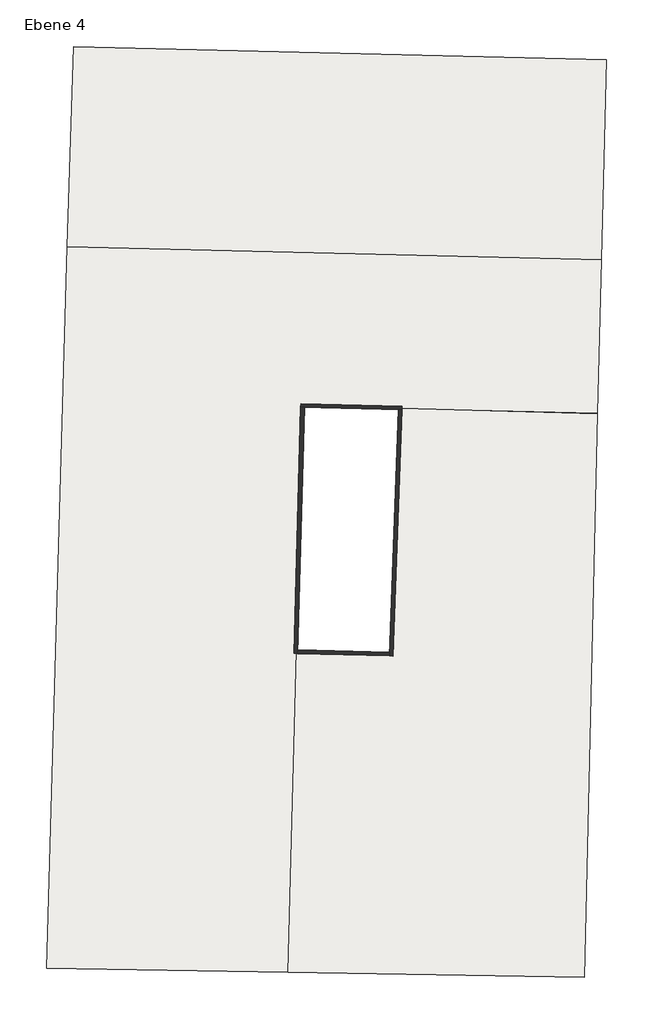
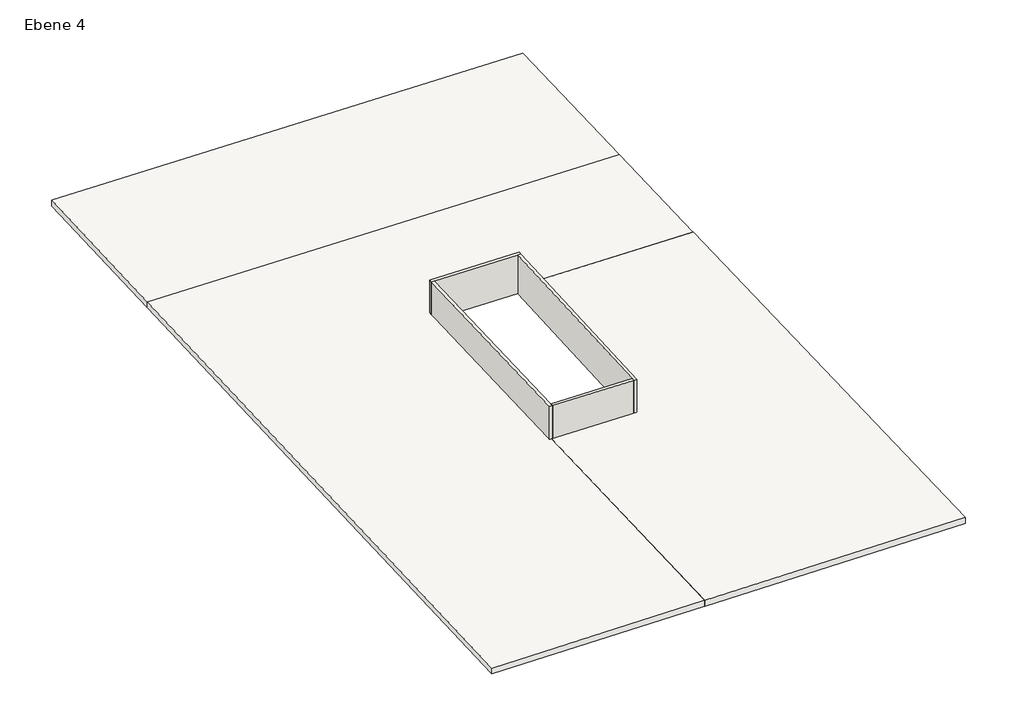
# One storey: 4 walls, 3 slabs.
"""IFC4 building model written with IfcOpenShell, lengths in millimetres."""

from ifc_helpers import new_model, si_unit, frame, origin, place, context, project, spatial, polyline, outline, extrude, faceted_brep, element, save

model = new_model("IFC4")

# Units and contexts
model_context = context("Model", 3, world=origin())
ifc_project = project(units=[si_unit("LENGTHUNIT", "METRE", prefix="MILLI")], contexts=[model_context])

# Site, building, storey
site = spatial("IfcSite", under=ifc_project)
building = spatial("IfcBuilding", under=site)
storey = spatial("IfcBuildingStorey", under=building, Name="Ebene 4", Elevation=3000.0)

# Slabs
placement = place(None, origin())
element("IfcSlab", 1, ObjectType="STB 20.0  FB 10.0 Akustikdecke", at=placement, inside=storey, context=model_context, shape_type="SweptSolid", body=[
    extrude(outline(polyline([(-1151.0631319, -18110.0518993), (-11455.315735, -17930.1905011), (-10568.7895571, 12833.151843), (12212.6461112, 12270.8579117), (12051.1906217, 5729.4608901), (-509.8782218, 6039.4945897), (-1151.0631319, -18110.0518993)])), frame((0.0, 0.0, 3000.0), z_axis=(0.0, 0.0, 1.0), x_axis=(1.0, 0.0, 0.0)), (0.0, 0.0, 1.0), 300.0),
])
element("IfcSlab", 2, ObjectType="STB 20.0  FB 10.0 Akustikdecke", at=placement, inside=storey, context=model_context, shape_type="SweptSolid", body=[
    extrude(outline(polyline([(11494.0304333, -18323.9009543), (-1144.0319966, -18103.302754), (-780.1414101, -4397.7515207), (3237.4967138, -4504.422217), (3618.3842953, 5943.1241384), (12050.8932593, 5719.2359795), (11494.0304333, -18323.9009543)])), frame((0.0, 0.0, 3000.0), z_axis=(0.0, 0.0, 1.0), x_axis=(1.0, 0.0, 0.0)), (0.0, 0.0, 1.0), 300.0),
])
element("IfcSlab", 3, ObjectType="STB 25.0  FB 10.0", at=placement, inside=storey, context=model_context, shape_type="SweptSolid", body=[
    extrude(outline(polyline([(12423.2323245, 20804.9758127), (12212.6461112, 12273.0390386), (-10562.4484458, 12835.1764579), (-10297.2009083, 21365.7640752), (12423.2323245, 20804.9758127)])), frame((0.0, 0.0, 3000.0), z_axis=(0.0, 0.0, 1.0), x_axis=(1.0, 0.0, 0.0)), (0.0, 0.0, 1.0), 300.0),
])

# Walls
element("IfcWall", 4, ObjectType="STB 10.0 + Akustikdecke", at=placement, inside=storey, context=model_context, shape_type="SweptSolid", body=[
    extrude(outline(polyline([(3179.0896913, -4616.4696663), (-735.4392226, -4512.5365812), (-731.4580358, -4362.5894234), (3184.5548982, -4466.5619101), (3179.0896913, -4616.4696663)])), frame((0.0, 0.0, 3000.0), z_axis=(0.0, 0.0, 1.0), x_axis=(1.0, 0.0, 0.0)), (0.0, 0.0, 1.0), 2000.0),
])
element("IfcWall", 5, ObjectType="STB 10.0 + Akustikdecke", at=placement, inside=storey, context=model_context, shape_type="Brep", body=[
    faceted_brep([(3329.0441926, -4620.451048, 3000.0), (3711.7017316, 5875.6443114, 3000.0), (3711.7017316, 5875.6443114, 5000.0), (3329.0441926, -4620.451048, 5000.0), (3179.0896913, -4616.4696663, 3000.0), (3179.0896913, -4616.4696663, 5000.0), (3184.5548982, -4466.5619101, 5000.0), (3561.7472302, 5879.6256932, 5000.0), (3561.7472302, 5879.6256932, 3000.0), (3184.5548982, -4466.5619101, 3000.0)], [[[0, 1, 2, 3]], [[4, 5, 6, 7, 8, 9]], [[0, 3, 5, 4]], [[1, 0, 4, 9, 8]], [[3, 2, 7, 6, 5]], [[2, 1, 8, 7]]]),
])
element("IfcWall", 6, ObjectType="STB 10.0 + Akustikdecke", at=placement, inside=storey, context=model_context, shape_type="Brep", body=[
    faceted_brep([(3717.1669385, 6025.5520677, 3000.0), (-602.6543337, 6140.2459074, 3000.0), (-602.6543337, 6140.2459074, 5000.0), (3717.1669385, 6025.5520677, 5000.0), (3711.7017316, 5875.6443114, 3000.0), (3711.7017316, 5875.6443114, 5000.0), (3561.7472302, 5879.6256932, 5000.0), (-456.6883626, 5986.3175627, 5000.0), (-606.6355205, 5990.2987495, 5000.0), (-606.6355205, 5990.2987495, 3000.0), (-456.6883626, 5986.3175627, 3000.0), (3561.7472302, 5879.6256932, 3000.0)], [[[0, 1, 2, 3]], [[4, 5, 6, 7, 8, 9, 10, 11]], [[1, 0, 4, 11, 10, 9]], [[3, 2, 8, 7, 6, 5]], [[0, 3, 5, 4]], [[2, 1, 9, 8]]]),
])
element("IfcWall", 7, ObjectType="STB 10.0 + Akustikdecke", at=placement, inside=storey, context=model_context, shape_type="Brep", body=[
    faceted_brep([(-606.6355205, 5990.2987495, 3000.0), (-885.3863804, -4508.5553945, 3000.0), (-885.3863804, -4508.5553945, 5000.0), (-606.6355205, 5990.2987495, 5000.0), (-456.6883626, 5986.3175627, 3000.0), (-456.6883626, 5986.3175627, 5000.0), (-731.4580358, -4362.5894234, 5000.0), (-735.4392226, -4512.5365812, 5000.0), (-735.4392226, -4512.5365812, 3000.0), (-731.4580358, -4362.5894234, 3000.0)], [[[0, 1, 2, 3]], [[4, 5, 6, 7, 8, 9]], [[1, 0, 4, 9, 8]], [[3, 2, 7, 6, 5]], [[2, 1, 8, 7]], [[0, 3, 5, 4]]]),
])

save(model, "model.ifc")

# Revit data of these elements
# Project information
#   Projektausgabedatum = "Projekt Datum"
#   Projektstatus = "Projektstatus"
#   Kundenname = "Bauherr"
#   Projektadresse = "Projektadresse"
#   Projektname = "Projektname"
#   Projektnummer = "Projektnummer"
#   Verfasser Firma 1 = "Firma 1"
#   Verfasser Firma 2 = "Firma 2"
#   Verfasser PLZ Ort = "PLZ Ort"
#   Verfasser Strasse = "Strasse"
#   Verfasser Telefon = "Telefon"
#   Verfasser Telefax = "Telefax"
#   Verfasser eMail = "E-Mail"
# Type "STB 20.0  FB 10.0 Akustikdecke"
#   Function = 0
#   Layers, outside or top first: 0.050 m "Standard - Fußboden" (function 4); 0.200 m "Stahlbeton - Ortbeton" (function 1); 0.050 m "Decke - Gipskarton" (function 4)
# Type "STB 25.0  FB 10.0"
#   Function = 0
#   Layers, outside or top first: 0.050 m "Standard - Fußboden" (function 4); 0.250 m "Stahlbeton - Ortbeton" (function 1)
# Type "STB 10.0 + Akustikdecke"
#   Type Comments = "Stahlbeton"
#   Description = "Stahlbeton 10.0"
#   Layers, outside or top first: 0.050 m "Decke - Gipskarton" (function 4); 0.100 m "Stahlbeton - Ortbeton" (function 1)
# Element 1 (IfcSlab, "STB 20.0  FB 10.0 Akustikdecke")
#   built-in parameter 1001955 = -1.59734 (stored number, unit not read)
#   Height Offset From Level = 0.300 m
#   built-in parameter 1001954 = 1
#   Phase Created = Phase 1
#   Materials on its faces: "Decke - Gipskarton", "Standard - Fußboden"
# Element 2 (IfcSlab, "STB 20.0  FB 10.0 Akustikdecke")
#   built-in parameter 1001955 = -1.59395 (stored number, unit not read)
#   Height Offset From Level = 0.300 m
#   Phase Created = Phase 1
#   Materials on its faces: "Decke - Gipskarton", "Standard - Fußboden"
# Element 3 (IfcSlab, "STB 25.0  FB 10.0")
#   Comments = ""
#   built-in parameter 1001955 = 1.54612 (stored number, unit not read)
#   Height Offset From Level = 0.300 m
#   built-in parameter 1001954 = 1
#   Phase Created = Phase 1
#   Materials on its faces: "Stahlbeton - Ortbeton", "Standard - Fußboden"
# Elements 4, 5, 7 (IfcWall, "STB 10.0 + Akustikdecke")
#   Comments = ""
#   Top Offset = 0.000 m
#   Base Offset = 0.000 m
#   wall height = 2.000 m
#   Phase Created = Phase 1
#   Base Constraint = Ebene 4
#   Top Constraint = Ebene 5
#   Materials on its faces: "Vorgabe - Wand", "Stahlbeton - Ortbeton", "Decke - Gipskarton"
# Element 6 (IfcWall, "STB 10.0 + Akustikdecke")
#   Comments = ""
#   Top Offset = 0.000 m
#   Base Offset = 0.000 m
#   wall height = 2.000 m
#   Phase Created = Phase 1
#   Base Constraint = Ebene 4
#   Top Constraint = Ebene 5
#   Materials on its faces: "Stahlbeton - Ortbeton", "Vorgabe - Wand", "Decke - Gipskarton"
# Materials
#   "Standard - Fußboden": class "Farbe 1", colour RGB 172 172 172, transparency 0, Cost = 0
#   "Stahlbeton - Ortbeton": class "Beton", colour RGB 192 192 192, transparency 0, Cost = 0
#   "Decke - Gipskarton": class "Trockenbauwand", colour RGB 255 255 255, transparency 0, Cost = 0
#   "Vorgabe - Wand": class "Stuck", colour RGB 53 53 53, transparency 0, Description = "Äußere Oberfläche", Cost = 0
